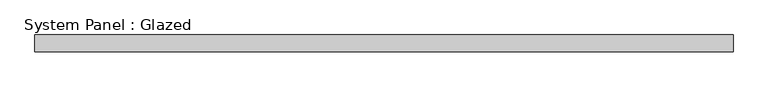
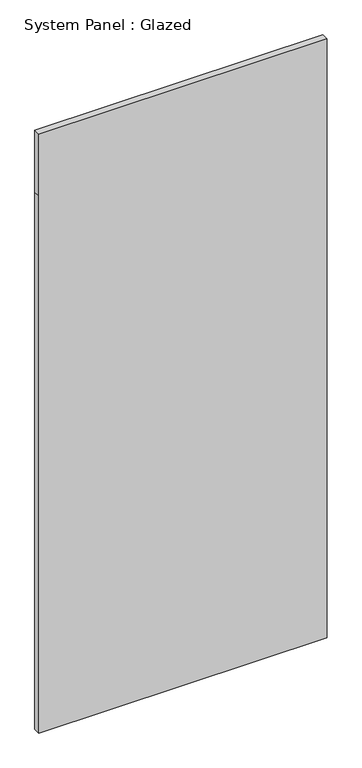
"""IFC4 building model written with IfcOpenShell, lengths in millimetres: plate geometry, System Panel : Glazed."""

from ifc_helpers import new_model, si_unit, frame, origin, place, context, project, spatial, polyline, outline, extrude, source, transform, mapped, element, save


def system_panel_glazed_011a4f1d(model_context):
    return source(origin(), model_context, "Body", "SweptSolid", [
        extrude(outline(polyline([(0.0, -533.4), (0.0, 533.4), (2101.85, 533.4), (2343.15, 533.4), (2343.15, -533.4), (2101.85, -533.4), (0.0, -533.4)])), frame((0.0, 19.05, 0.0), z_axis=(0.0, 1.0, 0.0), x_axis=(0.0, 0.0, 1.0)), (0.0, 0.0, 1.0), 25.4),
    ])


if __name__ == "__main__":
    model = new_model("IFC4")
    model_context = context("Model", 3, world=origin())
    ifc_project = project(units=[si_unit("LENGTHUNIT", "METRE", prefix="MILLI")], contexts=[model_context])
    site = spatial("IfcSite", under=ifc_project)
    building = spatial("IfcBuilding", under=site)
    placement = place(None, origin())
    system_panel_glazed_shape = system_panel_glazed_011a4f1d(model_context)
    element("IfcPlate", 1, ObjectType="System Panel : Glazed", at=placement, inside=building, context=model_context, shape_type="MappedRepresentation", body=[
        mapped(system_panel_glazed_shape, transform((0.0, 0.0, 0.0), x_axis=(1.0, 0.0, 0.0), y_axis=(0.0, 1.0, 0.0), z_axis=(0.0, 0.0, 1.0))),
    ])
    save(model, "model.ifc")

# Revit data of these elements
# Element 1 (IfcPlate, "System Panel : Glazed")
#   Materials on its faces: "Glass"
# Materials
#   "Glass": class "Glass", colour RGB 0 128 192, transparency 0.75
